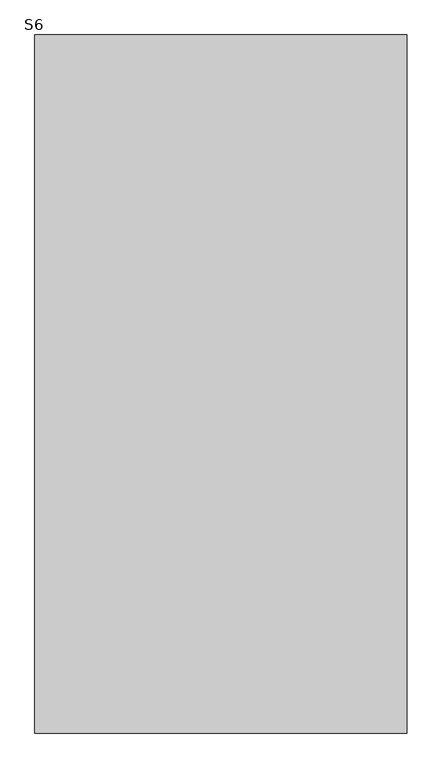
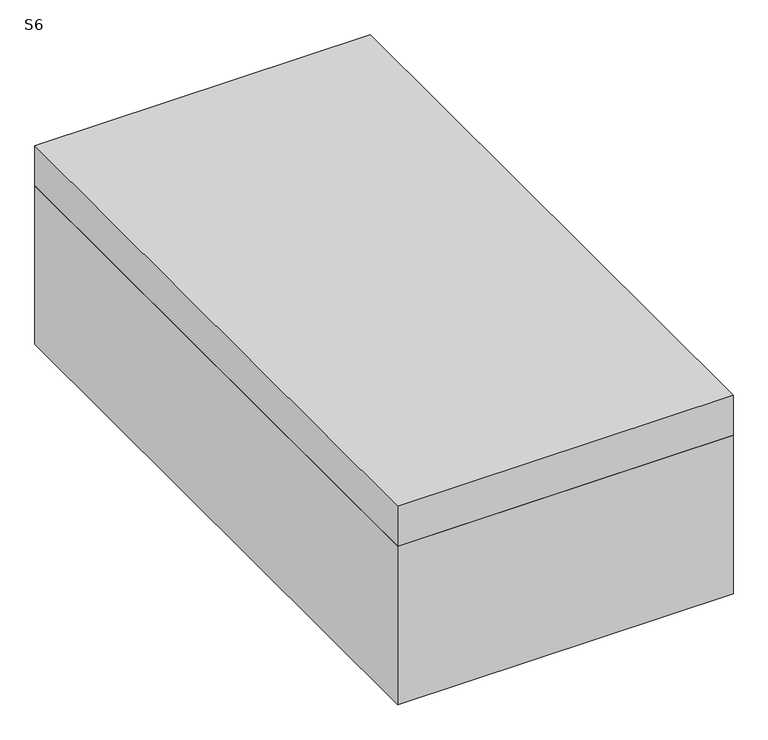
"""IFC4 building model written with IfcOpenShell, lengths in millimetres: fastener geometry, TQS - Sapata : S6."""

import ifcopenshell
import ifcopenshell.guid

model = None  # the IFC model being written
_history = None  # IfcOwnerHistory: only IFC2X3 demands one
_inside = {}  # id of a spatial element -> (the spatial element, [elements in it])
_under = {}  # id of a project, library or spatial element -> (it, [spatial elements below it])
_declared = {}  # id of a project -> (the project, [libraries it declares])
_typed = {}  # id of a type object -> (the type object, [elements of that type])
_made_of = {}  # id of a material, layer set ... -> (it, [elements and type objects made of it])


def new_model(schema):
    """Start an empty IFC model of exactly this schema.

    Asked for "IFC4X3", IfcOpenShell would pick the latest addendum, in which some entities
    have other attributes; the version numbers below select the first issue.
    IFC2X3 requires an IfcOwnerHistory on every rooted entity: one is made here for all.
    """
    global model, _history
    if schema == "IFC4X3":
        model = ifcopenshell.file(schema_version=(4, 3, 0, 0))
    else:
        model = ifcopenshell.file(schema=schema)
    _inside.clear()
    _under.clear()
    _declared.clear()
    _typed.clear()
    _made_of.clear()
    _history = None
    if model.schema == "IFC2X3":
        org = make("IfcOrganization", Name="unknown")
        user = make(
            "IfcPersonAndOrganization",
            ThePerson=make("IfcPerson", FamilyName="unknown"),
            TheOrganization=org,
        )
        app = make(
            "IfcApplication",
            ApplicationDeveloper=org,
            Version="unknown",
            ApplicationFullName="unknown",
            ApplicationIdentifier="unknown",
        )
        _history = make(
            "IfcOwnerHistory",
            OwningUser=user,
            OwningApplication=app,
            ChangeAction="ADDED",
            CreationDate=0,
        )
    return model


def make(cls, **values):
    """One entity of the class cls with the attributes given. An attribute that is None is left unset."""
    return model.create_entity(
        cls, **{name: value for name, value in values.items() if value is not None}
    )


def rooted(cls, **values):
    """An entity with a GlobalId (a new one), such as an element, a storey or a relation."""
    return make(cls, GlobalId=ifcopenshell.guid.new(), OwnerHistory=_history, **values)


def si_unit(unit_type, name, prefix=None):
    """IfcSIUnit, for example si_unit("LENGTHUNIT", "METRE", prefix="MILLI")."""
    return make("IfcSIUnit", UnitType=unit_type, Prefix=prefix, Name=name)


def assignment(units):
    """IfcUnitAssignment: the units of a project."""
    return None if units is None else make("IfcUnitAssignment", Units=units)


def point(xyz):
    """IfcCartesianPoint."""
    return None if xyz is None else make("IfcCartesianPoint", Coordinates=xyz)


def direction(xyz):
    """IfcDirection."""
    return None if xyz is None else make("IfcDirection", DirectionRatios=xyz)


def frame(location, z_axis=None, x_axis=None):
    """IfcAxis2Placement3D, a coordinate frame: its origin and axes. An axis left out is left unset."""
    return make(
        "IfcAxis2Placement3D",
        Location=point(location),
        Axis=direction(z_axis),
        RefDirection=direction(x_axis),
    )


def origin():
    """The frame at (0, 0, 0) with its axes left unset."""
    return frame((0.0, 0.0, 0.0))


def place(relative_to, where):
    """IfcLocalPlacement: puts the frame where relative to a parent placement (None: the world)."""
    return make(
        "IfcLocalPlacement", PlacementRelTo=relative_to, RelativePlacement=where
    )


def context(
    kind, dimensions, precision=None, world=None, true_north=None, identifier=None
):
    """IfcGeometricRepresentationContext, for example the 3D "Model" context."""
    return make(
        "IfcGeometricRepresentationContext",
        ContextIdentifier=identifier,
        ContextType=kind,
        CoordinateSpaceDimension=dimensions,
        Precision=precision,
        WorldCoordinateSystem=world,
        TrueNorth=true_north,
    )


def project(units=None, contexts=None):
    """IfcProject with its units and contexts."""
    return rooted(
        "IfcProject",
        Name="project",
        RepresentationContexts=contexts,
        UnitsInContext=assignment(units),
    )


def spatial(cls, under=None, at=None, **own):
    """A site, building, storey or space (cls), placed at a placement, below another one or the project."""
    s = rooted(cls, ObjectPlacement=at, **own)
    if under is not None:
        _under.setdefault(under.id(), (under, []))[1].append(s)
    return s


def polyline(points):
    """IfcPolyline through the points."""
    return make("IfcPolyline", Points=[point(p) for p in points])


def outline(outer, holes=None, kind="AREA"):
    """IfcArbitraryClosedProfileDef: a profile drawn as a closed curve; with holes, ...WithVoids."""
    if holes is None:
        return make("IfcArbitraryClosedProfileDef", ProfileType=kind, OuterCurve=outer)
    return make(
        "IfcArbitraryProfileDefWithVoids",
        ProfileType=kind,
        OuterCurve=outer,
        InnerCurves=holes,
    )


def extrude(swept, where, along, depth):
    """IfcExtrudedAreaSolid: the profile swept, set in the frame where, extruded along a direction by depth."""
    return make(
        "IfcExtrudedAreaSolid",
        SweptArea=swept,
        Position=where,
        ExtrudedDirection=direction(along),
        Depth=depth,
    )


def shape(context_of_items, identifier, shape_type, items):
    """IfcShapeRepresentation: the items that make up one representation, for example the "Body"."""
    return make(
        "IfcShapeRepresentation",
        ContextOfItems=context_of_items,
        RepresentationIdentifier=identifier,
        RepresentationType=shape_type,
        Items=items,
    )


def source(mapping_origin, context_of_items, identifier, shape_type, items):
    """IfcRepresentationMap: a shape defined once, which mapped items show again and again."""
    return make(
        "IfcRepresentationMap",
        MappingOrigin=mapping_origin,
        MappedRepresentation=shape(context_of_items, identifier, shape_type, items),
    )


def transform(
    local_origin,
    x_axis=None,
    y_axis=None,
    z_axis=None,
    scale=None,
    scale2=None,
    scale3=None,
    uniform=True,
):
    """IfcCartesianTransformationOperator3D, or its non-uniform kind. x_axis, y_axis, z_axis: its Axis1, 2, 3."""
    if uniform:
        return make(
            "IfcCartesianTransformationOperator3D",
            Axis1=direction(x_axis),
            Axis2=direction(y_axis),
            LocalOrigin=point(local_origin),
            Scale=scale,
            Axis3=direction(z_axis),
        )
    return make(
        "IfcCartesianTransformationOperator3DnonUniform",
        Axis1=direction(x_axis),
        Axis2=direction(y_axis),
        LocalOrigin=point(local_origin),
        Scale=scale,
        Axis3=direction(z_axis),
        Scale2=scale2,
        Scale3=scale3,
    )


def mapped(mapping_source, mapping_target):
    """IfcMappedItem: shows the shape of a source again, moved by a transform."""
    return make(
        "IfcMappedItem", MappingSource=mapping_source, MappingTarget=mapping_target
    )


def made_of(thing, what):
    """Note that an element or type object is made of a material, layer set ...; save() writes the relation."""
    if what is not None:
        _made_of.setdefault(what.id(), (what, []))[1].append(thing)
    return thing


def element(
    cls,
    number,
    at=None,
    inside=None,
    cuts=None,
    type_object=None,
    material=None,
    context=None,
    identifier="Body",
    shape_type=None,
    held_by="IfcProductDefinitionShape",
    body=None,
    shapes=None,
    **own,
):
    """One element of the class cls, such as IfcWall. Its Tag is "e" and its number.

    at: its placement. inside: the storey or other place that contains it. cuts: it is an
    opening in that element (IfcRelVoidsElement). A single representation is given by context,
    identifier, shape_type and body (its items); several are given by shapes. held_by: the class
    of the entity that holds the representations. save() writes the other relations.
    """
    e = rooted(cls, Tag="e%d" % number, ObjectPlacement=at, **own)
    if body is not None:
        shapes = [shape(context, identifier, shape_type, body)]
    if shapes is not None:
        e.Representation = make(held_by, Representations=shapes)
    if inside is not None:
        _inside.setdefault(inside.id(), (inside, []))[1].append(e)
    if cuts is not None:
        rooted(
            "IfcRelVoidsElement", RelatingBuildingElement=cuts, RelatedOpeningElement=e
        )
    if type_object is not None:
        _typed.setdefault(type_object.id(), (type_object, []))[1].append(e)
    return made_of(e, material)


def aggregate(whole, parts):
    """IfcRelAggregates: a whole, such as a stair, and the parts it consists of."""
    return rooted("IfcRelAggregates", RelatingObject=whole, RelatedObjects=parts)


def save(model, path):
    """Write the relations noted so far, then the file.

    IfcRelAggregates (storeys below a building ...), IfcRelContainedInSpatialStructure (elements
    in a storey), IfcRelDefinesByType, IfcRelAssociatesMaterial and IfcRelDeclares: one each for
    every whole, place, type object, material and project.
    """
    for whole, parts in _under.values():
        aggregate(whole, parts)
    for where, things in _inside.values():
        rooted(
            "IfcRelContainedInSpatialStructure",
            RelatedElements=things,
            RelatingStructure=where,
        )
    for kind, things in _typed.values():
        rooted("IfcRelDefinesByType", RelatedObjects=things, RelatingType=kind)
    for what, things in _made_of.values():
        rooted("IfcRelAssociatesMaterial", RelatedObjects=things, RelatingMaterial=what)
    for by, libraries in _declared.values():
        rooted("IfcRelDeclares", RelatingContext=by, RelatedDefinitions=libraries)
    model.write(path)


def s6_dd942dc6(model_context):
    return source(origin(), model_context, "Body", "SweptSolid", [
        extrude(outline(polyline([(200.0, 550.0), (200.0, -950.0), (-600.0, -950.0), (-600.0, 550.0), (200.0, 550.0)])), frame((0.0, 0.0, -100.0), z_axis=(0.0, 0.0, 1.0), x_axis=(1.0, 0.0, 0.0)), (0.0, 0.0, 1.0), 100.0),
        extrude(outline(polyline([(200.0, 550.0), (200.0, -950.0), (-600.0, -950.0), (-600.0, 550.0), (200.0, 550.0)])), frame((0.0, 0.0, -500.0), z_axis=(0.0, 0.0, 1.0), x_axis=(1.0, 0.0, 0.0)), (0.0, 0.0, 1.0), 400.0),
    ])


if __name__ == "__main__":
    model = new_model("IFC4")
    model_context = context("Model", 3, world=origin())
    ifc_project = project(units=[si_unit("LENGTHUNIT", "METRE", prefix="MILLI")], contexts=[model_context])
    site = spatial("IfcSite", under=ifc_project)
    building = spatial("IfcBuilding", under=site)
    placement = place(None, origin())
    s6_shape = s6_dd942dc6(model_context)
    element("IfcFastener", 1, ObjectType="TQS - Sapata : S6", at=placement, inside=building, context=model_context, shape_type="MappedRepresentation", body=[
        mapped(s6_shape, transform((0.0, 0.0, 0.0), x_axis=(1.0, 0.0, 0.0), y_axis=(0.0, 1.0, 0.0), z_axis=(0.0, 0.0, 1.0))),
    ])
    save(model, "model.ifc")

# Revit data of these elements
# Type "TQS - Sapata : S6"
#   TY = 1.50 m
#   TX = 0.80 m
#   HS = 0.50 m
#   H0 = 0.40 m
#   EXCYABS = 0.75 m
#   EXCY = 0.00 m
#   EXCXABS = 0.40 m
#   EXCX = 0.00 m
#   DIMY = 1.50 m
#   DIMX = 0.80 m
#   Material estrutural = Concreto - Concreto concretado no local
#   Width = 0
#   Length = 0
# Element 1 (IfcFastener, "TQS - Sapata : S6")
#   Materials on its faces: "Concreto - Concreto concretado no local"
# Materials
#   "Concreto - Concreto concretado no local": class "Concreto", colour RGB 192 192 192, transparency 0
